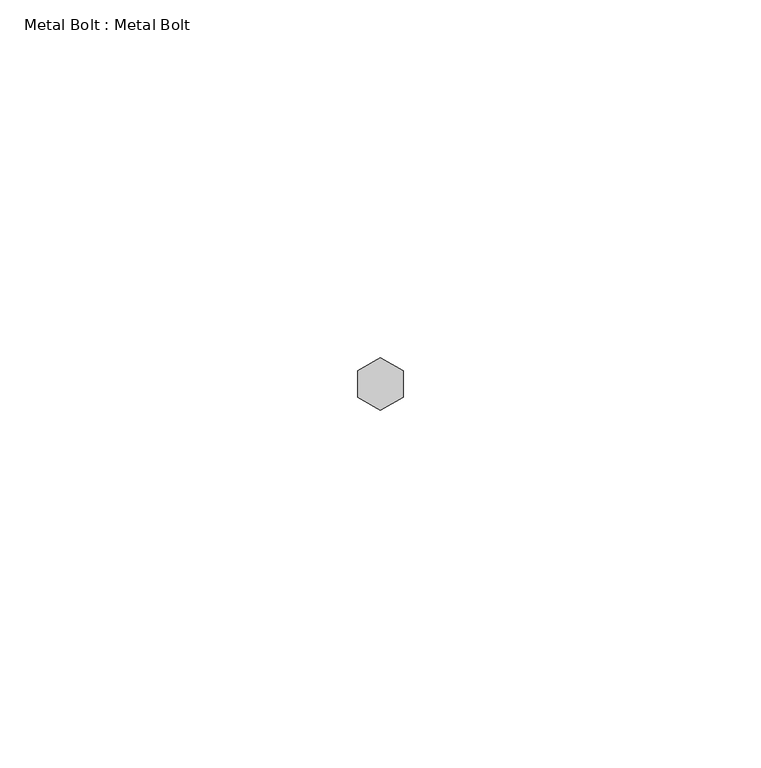
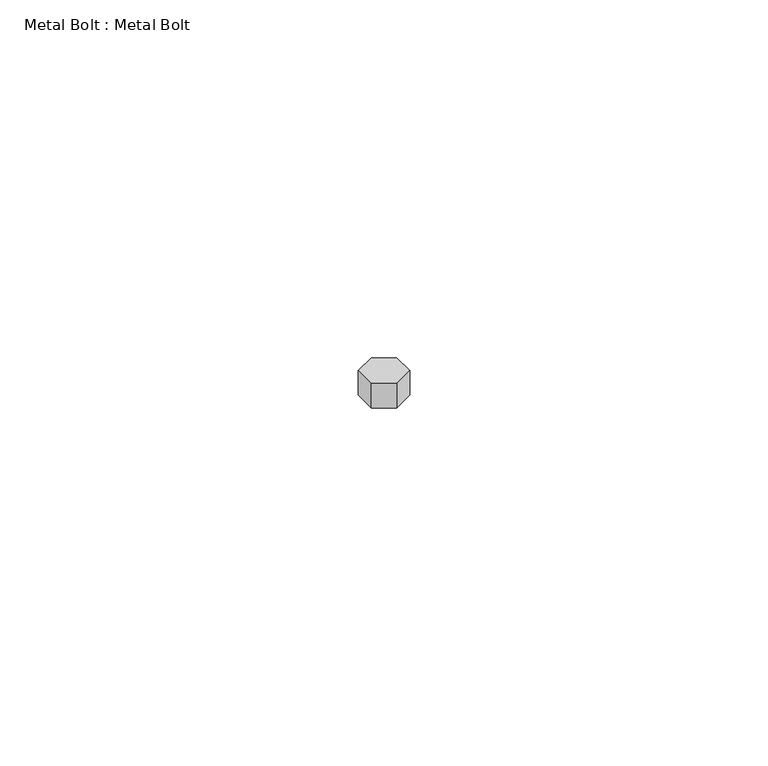
"""IFC4 building model written with IfcOpenShell, lengths in millimetres: proxy geometry, Metal Bolt : Metal Bolt."""

from ifc_helpers import new_model, si_unit, origin, origin_with_axes, place, context, project, spatial, polyline, outline, extrude, source, transform, mapped, element, save


def metal_bolt_metal_bolt_dc090140(model_context):
    return source(origin(), model_context, "Body", "SweptSolid", [
        extrude(outline(polyline([(-3.175, 1.8330871), (0.0, 3.6661742), (3.175, 1.8330871), (3.175, -1.8330871), (0.0, -3.6661742), (-3.175, -1.8330871), (-3.175, 1.8330871)])), origin_with_axes(), (0.0, 0.0, 1.0), 4.2333333),
    ])


if __name__ == "__main__":
    model = new_model("IFC4")
    model_context = context("Model", 3, world=origin())
    ifc_project = project(units=[si_unit("LENGTHUNIT", "METRE", prefix="MILLI")], contexts=[model_context])
    site = spatial("IfcSite", under=ifc_project)
    building = spatial("IfcBuilding", under=site)
    placement = place(None, origin())
    metal_bolt_metal_bolt_shape = metal_bolt_metal_bolt_dc090140(model_context)
    element("IfcBuildingElementProxy", 1, Name="Metal Bolt : Metal Bolt", ObjectType="Metal Bolt : Metal Bolt", at=placement, inside=building, context=model_context, shape_type="MappedRepresentation", body=[
        mapped(metal_bolt_metal_bolt_shape, transform((0.0, 0.0, 0.0), x_axis=(1.0, 0.0, 0.0), y_axis=(0.0, 1.0, 0.0), z_axis=(0.0, 0.0, 1.0))),
    ])
    save(model, "model.ifc")

# Revit data of these elements
# Type "Metal Bolt : Metal Bolt"
#   Height = 0' - 0.16667"
#   H2 = 0' - 0 1/2"
#   F3 = 0' - 0 1/16"
#   F2 = 0' - 0 1/8"
#   F = 0' - 0 1/4"
# Element 1 (IfcBuildingElementProxy, "Metal Bolt : Metal Bolt")
#   Materials on its faces: "UNISTRUT 1/4\" FIBERGLASS HEX FLANGED BOLT"
# Materials
#   "UNISTRUT 1/4\" FIBERGLASS HEX FLANGED BOLT": class "Miscellaneous", colour RGB 236 232 217, transparency 0, Cost = 0
